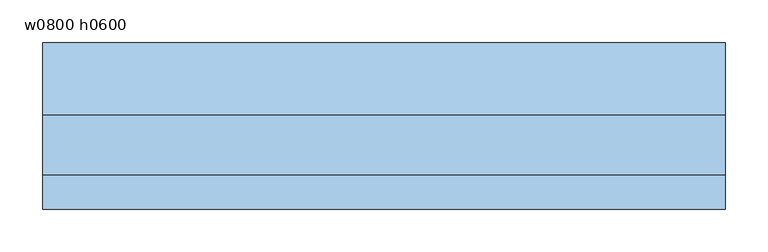
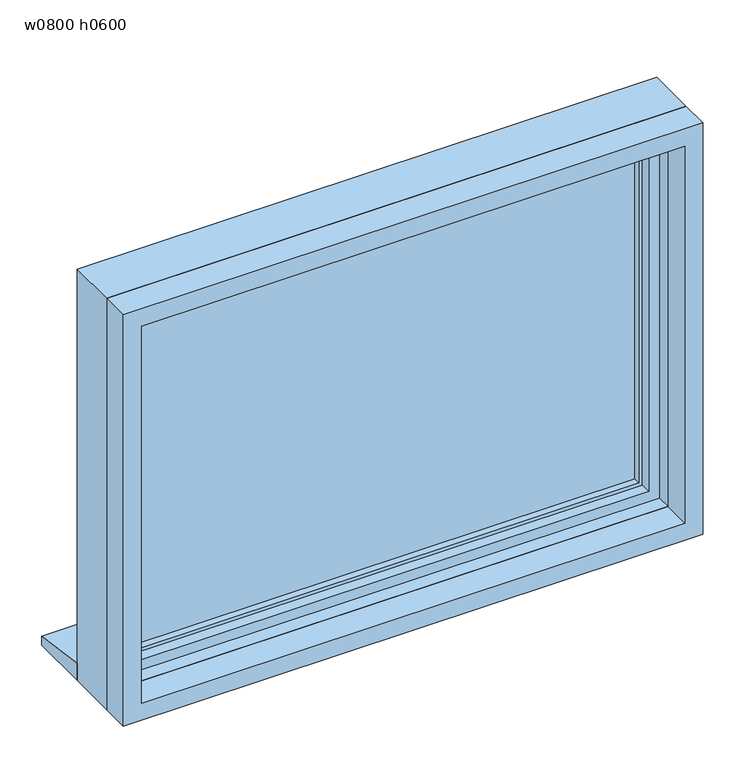
"""IFC4 building model written with IfcOpenShell, lengths in millimetres: window geometry, 突出し窓 : w0800 h0600."""

import ifcopenshell
import ifcopenshell.guid

model = None  # the IFC model being written
_history = None  # IfcOwnerHistory: only IFC2X3 demands one
_inside = {}  # id of a spatial element -> (the spatial element, [elements in it])
_under = {}  # id of a project, library or spatial element -> (it, [spatial elements below it])
_declared = {}  # id of a project -> (the project, [libraries it declares])
_typed = {}  # id of a type object -> (the type object, [elements of that type])
_made_of = {}  # id of a material, layer set ... -> (it, [elements and type objects made of it])


def new_model(schema):
    """Start an empty IFC model of exactly this schema.

    Asked for "IFC4X3", IfcOpenShell would pick the latest addendum, in which some entities
    have other attributes; the version numbers below select the first issue.
    IFC2X3 requires an IfcOwnerHistory on every rooted entity: one is made here for all.
    """
    global model, _history
    if schema == "IFC4X3":
        model = ifcopenshell.file(schema_version=(4, 3, 0, 0))
    else:
        model = ifcopenshell.file(schema=schema)
    _inside.clear()
    _under.clear()
    _declared.clear()
    _typed.clear()
    _made_of.clear()
    _history = None
    if model.schema == "IFC2X3":
        org = make("IfcOrganization", Name="unknown")
        user = make(
            "IfcPersonAndOrganization",
            ThePerson=make("IfcPerson", FamilyName="unknown"),
            TheOrganization=org,
        )
        app = make(
            "IfcApplication",
            ApplicationDeveloper=org,
            Version="unknown",
            ApplicationFullName="unknown",
            ApplicationIdentifier="unknown",
        )
        _history = make(
            "IfcOwnerHistory",
            OwningUser=user,
            OwningApplication=app,
            ChangeAction="ADDED",
            CreationDate=0,
        )
    return model


def make(cls, **values):
    """One entity of the class cls with the attributes given. An attribute that is None is left unset."""
    return model.create_entity(
        cls, **{name: value for name, value in values.items() if value is not None}
    )


def rooted(cls, **values):
    """An entity with a GlobalId (a new one), such as an element, a storey or a relation."""
    return make(cls, GlobalId=ifcopenshell.guid.new(), OwnerHistory=_history, **values)


def si_unit(unit_type, name, prefix=None):
    """IfcSIUnit, for example si_unit("LENGTHUNIT", "METRE", prefix="MILLI")."""
    return make("IfcSIUnit", UnitType=unit_type, Prefix=prefix, Name=name)


def assignment(units):
    """IfcUnitAssignment: the units of a project."""
    return None if units is None else make("IfcUnitAssignment", Units=units)


def point(xyz):
    """IfcCartesianPoint."""
    return None if xyz is None else make("IfcCartesianPoint", Coordinates=xyz)


def direction(xyz):
    """IfcDirection."""
    return None if xyz is None else make("IfcDirection", DirectionRatios=xyz)


def frame(location, z_axis=None, x_axis=None):
    """IfcAxis2Placement3D, a coordinate frame: its origin and axes. An axis left out is left unset."""
    return make(
        "IfcAxis2Placement3D",
        Location=point(location),
        Axis=direction(z_axis),
        RefDirection=direction(x_axis),
    )


def origin():
    """The frame at (0, 0, 0) with its axes left unset."""
    return frame((0.0, 0.0, 0.0))


def place(relative_to, where):
    """IfcLocalPlacement: puts the frame where relative to a parent placement (None: the world)."""
    return make(
        "IfcLocalPlacement", PlacementRelTo=relative_to, RelativePlacement=where
    )


def context(
    kind, dimensions, precision=None, world=None, true_north=None, identifier=None
):
    """IfcGeometricRepresentationContext, for example the 3D "Model" context."""
    return make(
        "IfcGeometricRepresentationContext",
        ContextIdentifier=identifier,
        ContextType=kind,
        CoordinateSpaceDimension=dimensions,
        Precision=precision,
        WorldCoordinateSystem=world,
        TrueNorth=true_north,
    )


def project(units=None, contexts=None):
    """IfcProject with its units and contexts."""
    return rooted(
        "IfcProject",
        Name="project",
        RepresentationContexts=contexts,
        UnitsInContext=assignment(units),
    )


def spatial(cls, under=None, at=None, **own):
    """A site, building, storey or space (cls), placed at a placement, below another one or the project."""
    s = rooted(cls, ObjectPlacement=at, **own)
    if under is not None:
        _under.setdefault(under.id(), (under, []))[1].append(s)
    return s


def polyline(points):
    """IfcPolyline through the points."""
    return make("IfcPolyline", Points=[point(p) for p in points])


def outline(outer, holes=None, kind="AREA"):
    """IfcArbitraryClosedProfileDef: a profile drawn as a closed curve; with holes, ...WithVoids."""
    if holes is None:
        return make("IfcArbitraryClosedProfileDef", ProfileType=kind, OuterCurve=outer)
    return make(
        "IfcArbitraryProfileDefWithVoids",
        ProfileType=kind,
        OuterCurve=outer,
        InnerCurves=holes,
    )


def extrude(swept, where, along, depth):
    """IfcExtrudedAreaSolid: the profile swept, set in the frame where, extruded along a direction by depth."""
    return make(
        "IfcExtrudedAreaSolid",
        SweptArea=swept,
        Position=where,
        ExtrudedDirection=direction(along),
        Depth=depth,
    )


def faces_of(points, faces, orient=None, outer=None):
    """IfcFace entities. A face is a list of loops; a loop is a list of indices into points, from 0.

    orient and outer hold one flag for each loop. By default every Orientation is true, the
    first loop of a face is its IfcFaceOuterBound and the others are IfcFaceBound.
    """
    made = []
    for i, loops in enumerate(faces):
        bounds = []
        for j, loop in enumerate(loops):
            is_outer = j == 0 if outer is None else outer[i][j]
            bounds.append(
                make(
                    "IfcFaceOuterBound" if is_outer else "IfcFaceBound",
                    Bound=make("IfcPolyLoop", Polygon=[points[k] for k in loop]),
                    Orientation=True if orient is None else orient[i][j],
                )
            )
        made.append(make("IfcFace", Bounds=bounds))
    return made


def faceted_brep(points, faces, orient=None, outer=None, voids=None):
    """IfcFacetedBrep: a solid bounded by flat faces; with voids (closed shells), ...WithVoids."""
    shared = [point(p) for p in points]
    hull = make("IfcClosedShell", CfsFaces=faces_of(shared, faces, orient, outer))
    if voids is None:
        return make("IfcFacetedBrep", Outer=hull)
    return make(
        "IfcFacetedBrepWithVoids",
        Outer=hull,
        Voids=[
            make(cls, CfsFaces=faces_of(shared, fs, o, b)) for cls, fs, o, b in voids
        ],
    )


def shape(context_of_items, identifier, shape_type, items):
    """IfcShapeRepresentation: the items that make up one representation, for example the "Body"."""
    return make(
        "IfcShapeRepresentation",
        ContextOfItems=context_of_items,
        RepresentationIdentifier=identifier,
        RepresentationType=shape_type,
        Items=items,
    )


def source(mapping_origin, context_of_items, identifier, shape_type, items):
    """IfcRepresentationMap: a shape defined once, which mapped items show again and again."""
    return make(
        "IfcRepresentationMap",
        MappingOrigin=mapping_origin,
        MappedRepresentation=shape(context_of_items, identifier, shape_type, items),
    )


def transform(
    local_origin,
    x_axis=None,
    y_axis=None,
    z_axis=None,
    scale=None,
    scale2=None,
    scale3=None,
    uniform=True,
):
    """IfcCartesianTransformationOperator3D, or its non-uniform kind. x_axis, y_axis, z_axis: its Axis1, 2, 3."""
    if uniform:
        return make(
            "IfcCartesianTransformationOperator3D",
            Axis1=direction(x_axis),
            Axis2=direction(y_axis),
            LocalOrigin=point(local_origin),
            Scale=scale,
            Axis3=direction(z_axis),
        )
    return make(
        "IfcCartesianTransformationOperator3DnonUniform",
        Axis1=direction(x_axis),
        Axis2=direction(y_axis),
        LocalOrigin=point(local_origin),
        Scale=scale,
        Axis3=direction(z_axis),
        Scale2=scale2,
        Scale3=scale3,
    )


def mapped(mapping_source, mapping_target):
    """IfcMappedItem: shows the shape of a source again, moved by a transform."""
    return make(
        "IfcMappedItem", MappingSource=mapping_source, MappingTarget=mapping_target
    )


def made_of(thing, what):
    """Note that an element or type object is made of a material, layer set ...; save() writes the relation."""
    if what is not None:
        _made_of.setdefault(what.id(), (what, []))[1].append(thing)
    return thing


def element(
    cls,
    number,
    at=None,
    inside=None,
    cuts=None,
    type_object=None,
    material=None,
    context=None,
    identifier="Body",
    shape_type=None,
    held_by="IfcProductDefinitionShape",
    body=None,
    shapes=None,
    **own,
):
    """One element of the class cls, such as IfcWall. Its Tag is "e" and its number.

    at: its placement. inside: the storey or other place that contains it. cuts: it is an
    opening in that element (IfcRelVoidsElement). A single representation is given by context,
    identifier, shape_type and body (its items); several are given by shapes. held_by: the class
    of the entity that holds the representations. save() writes the other relations.
    """
    e = rooted(cls, Tag="e%d" % number, ObjectPlacement=at, **own)
    if body is not None:
        shapes = [shape(context, identifier, shape_type, body)]
    if shapes is not None:
        e.Representation = make(held_by, Representations=shapes)
    if inside is not None:
        _inside.setdefault(inside.id(), (inside, []))[1].append(e)
    if cuts is not None:
        rooted(
            "IfcRelVoidsElement", RelatingBuildingElement=cuts, RelatedOpeningElement=e
        )
    if type_object is not None:
        _typed.setdefault(type_object.id(), (type_object, []))[1].append(e)
    return made_of(e, material)


def aggregate(whole, parts):
    """IfcRelAggregates: a whole, such as a stair, and the parts it consists of."""
    return rooted("IfcRelAggregates", RelatingObject=whole, RelatedObjects=parts)


def save(model, path):
    """Write the relations noted so far, then the file.

    IfcRelAggregates (storeys below a building ...), IfcRelContainedInSpatialStructure (elements
    in a storey), IfcRelDefinesByType, IfcRelAssociatesMaterial and IfcRelDeclares: one each for
    every whole, place, type object, material and project.
    """
    for whole, parts in _under.values():
        aggregate(whole, parts)
    for where, things in _inside.values():
        rooted(
            "IfcRelContainedInSpatialStructure",
            RelatedElements=things,
            RelatingStructure=where,
        )
    for kind, things in _typed.values():
        rooted("IfcRelDefinesByType", RelatedObjects=things, RelatingType=kind)
    for what, things in _made_of.values():
        rooted("IfcRelAssociatesMaterial", RelatedObjects=things, RelatingMaterial=what)
    for by, libraries in _declared.values():
        rooted("IfcRelDeclares", RelatingContext=by, RelatedDefinitions=libraries)
    model.write(path)


def w0800_h0600_72c0e8ae(model_context):
    return source(origin(), model_context, "Body", "SolidModel", [
        faceted_brep([(-400.0, -45.0, 1400.0), (-400.0, 25.0, 1400.0), (-400.0, 25.0, 800.0), (-400.0, -45.0, 800.0), (400.0, 25.0, 1400.0), (400.0, 25.0, 800.0), (-375.0, 25.0, 825.0), (375.0, 25.0, 825.0), (375.0, 25.0, 1375.0), (-375.0, 25.0, 1375.0), (400.0, -45.0, 800.0), (400.0, -45.0, 1400.0), (-375.0, -45.0, 1375.0), (375.0, -45.0, 1375.0), (375.0, -45.0, 825.0), (-375.0, -45.0, 825.0), (-375.0, -25.0, 1375.0), (-375.0, -25.0, 825.0), (375.0, -25.0, 825.0), (375.0, -25.0, 1375.0), (-360.0, -25.0, 1360.0), (360.0, -25.0, 1360.0), (360.0, -25.0, 840.0), (-360.0, -25.0, 840.0), (-360.0, -10.0, 1360.0), (-360.0, -10.0, 840.0), (360.0, -10.0, 840.0), (-375.0, -10.0, 1375.0), (375.0, -10.0, 1375.0), (375.0, -10.0, 825.0), (-375.0, -10.0, 825.0), (360.0, -10.0, 1360.0)], [[[0, 1, 2, 3]], [[1, 4, 5, 2], [6, 7, 8, 9]], [[3, 2, 5, 10]], [[3, 10, 11, 0], [12, 13, 14, 15]], [[16, 12, 15, 17]], [[17, 15, 14, 18]], [[17, 18, 19, 16], [20, 21, 22, 23]], [[24, 20, 23, 25]], [[25, 23, 22, 26]], [[27, 28, 29, 30], [25, 26, 31, 24]], [[9, 27, 30, 6]], [[6, 30, 29, 7]], [[10, 5, 4, 11]], [[18, 14, 13, 19]], [[26, 22, 21, 31]], [[7, 29, 28, 8]], [[11, 4, 1, 0]], [[19, 13, 12, 16]], [[31, 21, 20, 24]], [[8, 28, 27, 9]]]),
        extrude(outline(polyline([(1400.0, 400.0), (1400.0, -400.0), (800.0, -400.0), (800.0, 400.0), (1400.0, 400.0)]), holes=[polyline([(825.0, 375.0), (825.0, -375.0), (1375.0, -375.0), (1375.0, 375.0), (825.0, 375.0)])]), frame((0.0, -85.0, 0.0), z_axis=(0.0, 1.0, 0.0), x_axis=(0.0, 0.0, 1.0)), (0.0, 0.0, 1.0), 40.0),
        extrude(outline(polyline([(355.0, 0.0), (-355.0, 0.0), (-355.0, 5.0), (355.0, 5.0), (355.0, 0.0)])), frame((0.0, 0.0, 845.0), z_axis=(0.0, 0.0, 1.0), x_axis=(1.0, 0.0, 0.0)), (0.0, 0.0, 1.0), 510.0),
        extrude(outline(polyline([(1375.0, 375.0), (1375.0, -375.0), (825.0, -375.0), (825.0, 375.0), (1375.0, 375.0)]), holes=[polyline([(1355.0, -355.0), (1355.0, 355.0), (845.0, 355.0), (845.0, -355.0), (1355.0, -355.0)])]), frame((0.0, -10.0, 0.0), z_axis=(0.0, 1.0, 0.0), x_axis=(0.0, 0.0, 1.0)), (0.0, 0.0, 1.0), 25.0),
        extrude(outline(polyline([(25.0, 800.0), (25.0, 825.0), (110.0, 813.0), (110.0, 800.0), (25.0, 800.0)])), frame((-400.0, 0.0, 0.0), z_axis=(1.0, 0.0, 0.0), x_axis=(0.0, 1.0, 0.0)), (0.0, 0.0, 1.0), 800.0),
    ])


if __name__ == "__main__":
    model = new_model("IFC4")
    model_context = context("Model", 3, world=origin())
    ifc_project = project(units=[si_unit("LENGTHUNIT", "METRE", prefix="MILLI")], contexts=[model_context])
    site = spatial("IfcSite", under=ifc_project)
    building = spatial("IfcBuilding", under=site)
    placement = place(None, origin())
    w0800_h0600_shape = w0800_h0600_72c0e8ae(model_context)
    element("IfcWindow", 1, ObjectType="突出し窓 : w0800 h0600", at=placement, inside=building, context=model_context, shape_type="MappedRepresentation", body=[
        mapped(w0800_h0600_shape, transform((0.0, 0.0, 0.0), x_axis=(1.0, 0.0, 0.0), y_axis=(0.0, 1.0, 0.0), z_axis=(0.0, 0.0, 1.0))),
    ])
    save(model, "model.ifc")

# Revit data of these elements
# Type "突出し窓 : w0800 h0600"
#   Construction Type Id = "GSP4R"
#   Analytic Construction = "1/8 インチ ピルキントン一重ガラス"
#   Type Mark = "99"
#   Operation = "シングルパネル"
#   Keynote = "08520.AA2"
#   Visual Light Transmittance = 0.9
#   Solar Heat Gain Coefficient = 0.86
#   Heat Transfer Coefficient (U) = 6.7069 W/(m²·K)
#   Height = 600 mm
#   額縁見附 = 25 mm
#   額縁ちり = 10 mm
#   既定の腰高 = 800 mm
#   Width = 800 mm
#   サッシ枠見附 = 40 mm
#   サッシ枠見込 = 70 mm
#   内枠 = 木目 - ナチュラル
#   サッシ = none
#   ガラス = ガラス - 透明
#   Wall Closure = (empty or 0)
# Element 1 (IfcWindow, "突出し窓 : w0800 h0600")
#   Materials on its faces: "木目 - ナチュラル", "ガラス - 透明"
# Materials
#   "木目 - ナチュラル": class "木材", colour RGB 204 173 122, transparency 0, Cost = 0
#   "ガラス - 透明": class "ガラス", colour RGB 0 128 192, transparency 0.9, Cost = 0
